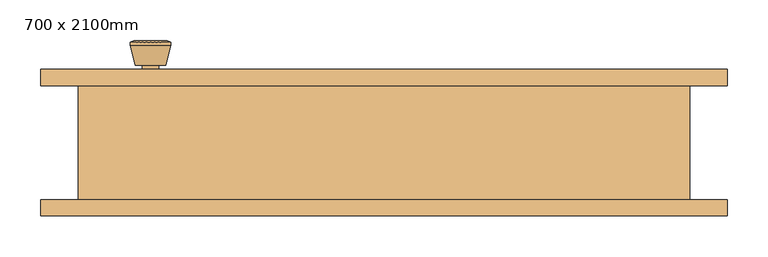
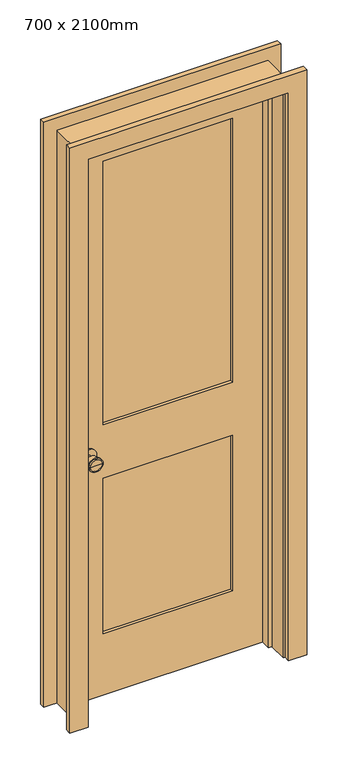
"""IFC4 building model written with IfcOpenShell, lengths in millimetres: door geometry, Porta-Interna-Única-2_Painel-Madeira : 700 x 2100mm."""

import ifcopenshell
import ifcopenshell.guid

model = None  # the IFC model being written
_history = None  # IfcOwnerHistory: only IFC2X3 demands one
_inside = {}  # id of a spatial element -> (the spatial element, [elements in it])
_under = {}  # id of a project, library or spatial element -> (it, [spatial elements below it])
_declared = {}  # id of a project -> (the project, [libraries it declares])
_typed = {}  # id of a type object -> (the type object, [elements of that type])
_made_of = {}  # id of a material, layer set ... -> (it, [elements and type objects made of it])


def new_model(schema):
    """Start an empty IFC model of exactly this schema.

    Asked for "IFC4X3", IfcOpenShell would pick the latest addendum, in which some entities
    have other attributes; the version numbers below select the first issue.
    IFC2X3 requires an IfcOwnerHistory on every rooted entity: one is made here for all.
    """
    global model, _history
    if schema == "IFC4X3":
        model = ifcopenshell.file(schema_version=(4, 3, 0, 0))
    else:
        model = ifcopenshell.file(schema=schema)
    _inside.clear()
    _under.clear()
    _declared.clear()
    _typed.clear()
    _made_of.clear()
    _history = None
    if model.schema == "IFC2X3":
        org = make("IfcOrganization", Name="unknown")
        user = make(
            "IfcPersonAndOrganization",
            ThePerson=make("IfcPerson", FamilyName="unknown"),
            TheOrganization=org,
        )
        app = make(
            "IfcApplication",
            ApplicationDeveloper=org,
            Version="unknown",
            ApplicationFullName="unknown",
            ApplicationIdentifier="unknown",
        )
        _history = make(
            "IfcOwnerHistory",
            OwningUser=user,
            OwningApplication=app,
            ChangeAction="ADDED",
            CreationDate=0,
        )
    return model


def make(cls, **values):
    """One entity of the class cls with the attributes given. An attribute that is None is left unset."""
    return model.create_entity(
        cls, **{name: value for name, value in values.items() if value is not None}
    )


def rooted(cls, **values):
    """An entity with a GlobalId (a new one), such as an element, a storey or a relation."""
    return make(cls, GlobalId=ifcopenshell.guid.new(), OwnerHistory=_history, **values)


def si_unit(unit_type, name, prefix=None):
    """IfcSIUnit, for example si_unit("LENGTHUNIT", "METRE", prefix="MILLI")."""
    return make("IfcSIUnit", UnitType=unit_type, Prefix=prefix, Name=name)


def assignment(units):
    """IfcUnitAssignment: the units of a project."""
    return None if units is None else make("IfcUnitAssignment", Units=units)


def point(xyz):
    """IfcCartesianPoint."""
    return None if xyz is None else make("IfcCartesianPoint", Coordinates=xyz)


def direction(xyz):
    """IfcDirection."""
    return None if xyz is None else make("IfcDirection", DirectionRatios=xyz)


def frame(location, z_axis=None, x_axis=None):
    """IfcAxis2Placement3D, a coordinate frame: its origin and axes. An axis left out is left unset."""
    return make(
        "IfcAxis2Placement3D",
        Location=point(location),
        Axis=direction(z_axis),
        RefDirection=direction(x_axis),
    )


def frame_2d(location, x_axis=None):
    """IfcAxis2Placement2D, a coordinate frame in the plane: its origin and x axis."""
    return make(
        "IfcAxis2Placement2D", Location=point(location), RefDirection=direction(x_axis)
    )


def origin():
    """The frame at (0, 0, 0) with its axes left unset."""
    return frame((0.0, 0.0, 0.0))


def place(relative_to, where):
    """IfcLocalPlacement: puts the frame where relative to a parent placement (None: the world)."""
    return make(
        "IfcLocalPlacement", PlacementRelTo=relative_to, RelativePlacement=where
    )


def context(
    kind, dimensions, precision=None, world=None, true_north=None, identifier=None
):
    """IfcGeometricRepresentationContext, for example the 3D "Model" context."""
    return make(
        "IfcGeometricRepresentationContext",
        ContextIdentifier=identifier,
        ContextType=kind,
        CoordinateSpaceDimension=dimensions,
        Precision=precision,
        WorldCoordinateSystem=world,
        TrueNorth=true_north,
    )


def project(units=None, contexts=None):
    """IfcProject with its units and contexts."""
    return rooted(
        "IfcProject",
        Name="project",
        RepresentationContexts=contexts,
        UnitsInContext=assignment(units),
    )


def spatial(cls, under=None, at=None, **own):
    """A site, building, storey or space (cls), placed at a placement, below another one or the project."""
    s = rooted(cls, ObjectPlacement=at, **own)
    if under is not None:
        _under.setdefault(under.id(), (under, []))[1].append(s)
    return s


def polyline(points):
    """IfcPolyline through the points."""
    return make("IfcPolyline", Points=[point(p) for p in points])


def circle_curve(where, radius):
    """IfcCircle in the frame where."""
    return make("IfcCircle", Position=where, Radius=radius)


def trimmed(basis, trim1, trim2, sense, master):
    """IfcTrimmedCurve: the piece of a basis curve between two trims."""
    return make(
        "IfcTrimmedCurve",
        BasisCurve=basis,
        Trim1=trim1,
        Trim2=trim2,
        SenseAgreement=sense,
        MasterRepresentation=master,
    )


def segment(curve, same_sense, transition):
    """IfcCompositeCurveSegment."""
    return make(
        "IfcCompositeCurveSegment",
        Transition=transition,
        SameSense=same_sense,
        ParentCurve=curve,
    )


def composite_curve(segments, self_intersect=None):
    """IfcCompositeCurve: segments joined end to end."""
    return make("IfcCompositeCurve", Segments=segments, SelfIntersect=self_intersect)


def outline(outer, holes=None, kind="AREA"):
    """IfcArbitraryClosedProfileDef: a profile drawn as a closed curve; with holes, ...WithVoids."""
    if holes is None:
        return make("IfcArbitraryClosedProfileDef", ProfileType=kind, OuterCurve=outer)
    return make(
        "IfcArbitraryProfileDefWithVoids",
        ProfileType=kind,
        OuterCurve=outer,
        InnerCurves=holes,
    )


def extrude(swept, where, along, depth):
    """IfcExtrudedAreaSolid: the profile swept, set in the frame where, extruded along a direction by depth."""
    return make(
        "IfcExtrudedAreaSolid",
        SweptArea=swept,
        Position=where,
        ExtrudedDirection=direction(along),
        Depth=depth,
    )


def faces_of(points, faces, orient=None, outer=None):
    """IfcFace entities. A face is a list of loops; a loop is a list of indices into points, from 0.

    orient and outer hold one flag for each loop. By default every Orientation is true, the
    first loop of a face is its IfcFaceOuterBound and the others are IfcFaceBound.
    """
    made = []
    for i, loops in enumerate(faces):
        bounds = []
        for j, loop in enumerate(loops):
            is_outer = j == 0 if outer is None else outer[i][j]
            bounds.append(
                make(
                    "IfcFaceOuterBound" if is_outer else "IfcFaceBound",
                    Bound=make("IfcPolyLoop", Polygon=[points[k] for k in loop]),
                    Orientation=True if orient is None else orient[i][j],
                )
            )
        made.append(make("IfcFace", Bounds=bounds))
    return made


def faceted_brep(points, faces, orient=None, outer=None, voids=None):
    """IfcFacetedBrep: a solid bounded by flat faces; with voids (closed shells), ...WithVoids."""
    shared = [point(p) for p in points]
    hull = make("IfcClosedShell", CfsFaces=faces_of(shared, faces, orient, outer))
    if voids is None:
        return make("IfcFacetedBrep", Outer=hull)
    return make(
        "IfcFacetedBrepWithVoids",
        Outer=hull,
        Voids=[
            make(cls, CfsFaces=faces_of(shared, fs, o, b)) for cls, fs, o, b in voids
        ],
    )


def shape(context_of_items, identifier, shape_type, items):
    """IfcShapeRepresentation: the items that make up one representation, for example the "Body"."""
    return make(
        "IfcShapeRepresentation",
        ContextOfItems=context_of_items,
        RepresentationIdentifier=identifier,
        RepresentationType=shape_type,
        Items=items,
    )


def source(mapping_origin, context_of_items, identifier, shape_type, items):
    """IfcRepresentationMap: a shape defined once, which mapped items show again and again."""
    return make(
        "IfcRepresentationMap",
        MappingOrigin=mapping_origin,
        MappedRepresentation=shape(context_of_items, identifier, shape_type, items),
    )


def transform(
    local_origin,
    x_axis=None,
    y_axis=None,
    z_axis=None,
    scale=None,
    scale2=None,
    scale3=None,
    uniform=True,
):
    """IfcCartesianTransformationOperator3D, or its non-uniform kind. x_axis, y_axis, z_axis: its Axis1, 2, 3."""
    if uniform:
        return make(
            "IfcCartesianTransformationOperator3D",
            Axis1=direction(x_axis),
            Axis2=direction(y_axis),
            LocalOrigin=point(local_origin),
            Scale=scale,
            Axis3=direction(z_axis),
        )
    return make(
        "IfcCartesianTransformationOperator3DnonUniform",
        Axis1=direction(x_axis),
        Axis2=direction(y_axis),
        LocalOrigin=point(local_origin),
        Scale=scale,
        Axis3=direction(z_axis),
        Scale2=scale2,
        Scale3=scale3,
    )


def mapped(mapping_source, mapping_target):
    """IfcMappedItem: shows the shape of a source again, moved by a transform."""
    return make(
        "IfcMappedItem", MappingSource=mapping_source, MappingTarget=mapping_target
    )


def made_of(thing, what):
    """Note that an element or type object is made of a material, layer set ...; save() writes the relation."""
    if what is not None:
        _made_of.setdefault(what.id(), (what, []))[1].append(thing)
    return thing


def element(
    cls,
    number,
    at=None,
    inside=None,
    cuts=None,
    type_object=None,
    material=None,
    context=None,
    identifier="Body",
    shape_type=None,
    held_by="IfcProductDefinitionShape",
    body=None,
    shapes=None,
    **own,
):
    """One element of the class cls, such as IfcWall. Its Tag is "e" and its number.

    at: its placement. inside: the storey or other place that contains it. cuts: it is an
    opening in that element (IfcRelVoidsElement). A single representation is given by context,
    identifier, shape_type and body (its items); several are given by shapes. held_by: the class
    of the entity that holds the representations. save() writes the other relations.
    """
    e = rooted(cls, Tag="e%d" % number, ObjectPlacement=at, **own)
    if body is not None:
        shapes = [shape(context, identifier, shape_type, body)]
    if shapes is not None:
        e.Representation = make(held_by, Representations=shapes)
    if inside is not None:
        _inside.setdefault(inside.id(), (inside, []))[1].append(e)
    if cuts is not None:
        rooted(
            "IfcRelVoidsElement", RelatingBuildingElement=cuts, RelatedOpeningElement=e
        )
    if type_object is not None:
        _typed.setdefault(type_object.id(), (type_object, []))[1].append(e)
    return made_of(e, material)


def aggregate(whole, parts):
    """IfcRelAggregates: a whole, such as a stair, and the parts it consists of."""
    return rooted("IfcRelAggregates", RelatingObject=whole, RelatedObjects=parts)


def save(model, path):
    """Write the relations noted so far, then the file.

    IfcRelAggregates (storeys below a building ...), IfcRelContainedInSpatialStructure (elements
    in a storey), IfcRelDefinesByType, IfcRelAssociatesMaterial and IfcRelDeclares: one each for
    every whole, place, type object, material and project.
    """
    for whole, parts in _under.values():
        aggregate(whole, parts)
    for where, things in _inside.values():
        rooted(
            "IfcRelContainedInSpatialStructure",
            RelatedElements=things,
            RelatingStructure=where,
        )
    for kind, things in _typed.values():
        rooted("IfcRelDefinesByType", RelatedObjects=things, RelatingType=kind)
    for what, things in _made_of.values():
        rooted("IfcRelAssociatesMaterial", RelatedObjects=things, RelatingMaterial=what)
    for by, libraries in _declared.values():
        rooted("IfcRelDeclares", RelatingContext=by, RelatedDefinitions=libraries)
    model.write(path)


def plane_surface(at):
    """IfcPlane: the flat surface through the origin of the frame at, square to its z axis."""
    return make("IfcPlane", Position=at)


def cylinder_surface(at, radius):
    """IfcCylindricalSurface: all points at the distance radius from the z axis of the frame at."""
    return make("IfcCylindricalSurface", Position=at, Radius=radius)


def revolved_surface(curve, axis_point, axis_direction):
    """IfcSurfaceOfRevolution: the curve turned about the line through axis_point along axis_direction."""
    return make(
        "IfcSurfaceOfRevolution",
        SweptCurve=make("IfcArbitraryOpenProfileDef", ProfileType="CURVE", Curve=curve),
        AxisPosition=make("IfcAxis1Placement", Location=point(axis_point), Axis=direction(axis_direction)),
    )


def advanced_brep(points, edges, surfaces, faces):
    """IfcAdvancedBrep: a solid bounded by faces that lie on surfaces and meet in shared edges.

    An edge is (start, end): straight between two places in points (the first is 0);
    or (start, end, curve); or (start, end, curve, False) where it runs against its curve.
    A face is (place in surfaces, loops), or (place, loops, False) where it looks against
    its surface's normal. A loop lists edges by number (the first is 1), with a minus sign
    where the edge is run from its end to its start. The first loop is the outer one.
    """
    corners = [point(p) for p in points]
    vertices = [make("IfcVertexPoint", VertexGeometry=c) for c in corners]
    made = []
    for start, end, *more in edges:
        made.append(
            make(
                "IfcEdgeCurve",
                EdgeStart=vertices[start],
                EdgeEnd=vertices[end],
                EdgeGeometry=more[0] if more else make("IfcPolyline", Points=[corners[start], corners[end]]),
                SameSense=more[1] if len(more) > 1 else True,
            )
        )
    hull = []
    for where, loops, *sense in faces:
        bounds = []
        for j, loop in enumerate(loops):
            ring = [make("IfcOrientedEdge", EdgeElement=made[abs(k) - 1], Orientation=k > 0) for k in loop]
            bounds.append(
                make(
                    "IfcFaceOuterBound" if j == 0 else "IfcFaceBound",
                    Bound=make("IfcEdgeLoop", EdgeList=ring),
                    Orientation=True,
                )
            )
        hull.append(make("IfcAdvancedFace", Bounds=bounds, FaceSurface=surfaces[where], SameSense=sense[0] if sense else True))
    return make("IfcAdvancedBrep", Outer=make("IfcClosedShell", CfsFaces=hull))


def door_700_x_2100mm_663e0b52(model_context):
    return source(origin(), model_context, "Body", "SolidModel", [
        advanced_brep(
        [(-286.5, 25.825, 914.4), (-276.5, 25.825, 914.4), (-296.5, 25.825, 914.4), (-266.0241324, -23.175, 914.4), (-286.5, -23.175, 914.4), (-306.9758676, -23.175, 914.4), (-261.5, -21.3471319, 914.4), (-311.5, -21.3471319, 914.4), (-261.5, -17.8834537, 914.4), (-311.5, -17.8834537, 914.4), (-267.863764, 6.825, 914.4), (-305.136236, 6.825, 914.4), (-276.5, 6.825, 914.4), (-296.5, 6.825, 914.4)],
        [
            (0, 1),
            (1, 2, circle_curve(frame((-286.5, 25.825, 914.4), z_axis=(0.0, 1.0, 0.0), x_axis=(-1.0, 0.0, 0.0)), 10.0)),
            (2, 0),
            (2, 1, circle_curve(frame((-286.5, 25.825, 914.4), z_axis=(0.0, 1.0, 0.0), x_axis=(-1.0, 0.0, 0.0)), 10.0)),
            (3, 4),
            (4, 5),
            (5, 3, circle_curve(frame((-286.5, -23.175, 914.4), z_axis=(0.0, -1.0, 0.0), x_axis=(-1.0, 0.0, 0.0)), 20.4758676)),
            (3, 5, circle_curve(frame((-286.5, -23.175, 914.4), z_axis=(0.0, -1.0, 0.0), x_axis=(-1.0, 0.0, 0.0)), 20.4758676)),
            (6, 3),
            (5, 7),
            (7, 6, circle_curve(frame((-286.5, -21.3471319, 914.4), z_axis=(0.0, -1.0, 0.0), x_axis=(-1.0, 0.0, 0.0)), 25.0)),
            (6, 7, circle_curve(frame((-286.5, -21.3471319, 914.4), z_axis=(0.0, -1.0, 0.0), x_axis=(-1.0, 0.0, 0.0)), 25.0)),
            (8, 6),
            (7, 9),
            (9, 8, circle_curve(frame((-286.5, -17.8834537, 914.4), z_axis=(0.0, -1.0, 0.0), x_axis=(-1.0, 0.0, 0.0)), 25.0)),
            (8, 9, circle_curve(frame((-286.5, -17.8834537, 914.4), z_axis=(0.0, -1.0, 0.0), x_axis=(-1.0, 0.0, 0.0)), 25.0)),
            (10, 8),
            (9, 11),
            (11, 10, circle_curve(frame((-286.5, 6.825, 914.4), z_axis=(0.0, -1.0, 0.0), x_axis=(-1.0, 0.0, 0.0)), 18.636236)),
            (10, 11, circle_curve(frame((-286.5, 6.825, 914.4), z_axis=(0.0, -1.0, 0.0), x_axis=(-1.0, 0.0, 0.0)), 18.636236)),
            (12, 10),
            (11, 13),
            (13, 12, circle_curve(frame((-286.5, 6.825, 914.4), z_axis=(0.0, -1.0, 0.0), x_axis=(-1.0, 0.0, 0.0)), 10.0)),
            (12, 13, circle_curve(frame((-286.5, 6.825, 914.4), z_axis=(0.0, -1.0, 0.0), x_axis=(-1.0, 0.0, 0.0)), 10.0)),
            (1, 12),
            (13, 2),
        ],
        [
            plane_surface(frame((-286.5, 25.825, 914.4), z_axis=(0.0, 1.0, 0.0), x_axis=(-1.0, 0.0, 0.0))),
            plane_surface(frame((-286.5, -23.175, 914.4), z_axis=(0.0, -1.0, 0.0), x_axis=(-1.0, 0.0, 0.0))),
            revolved_surface(polyline([(-306.9758676, -23.175, 914.4), (-311.5, -21.3471319, 914.4)]), (-286.5, 25.825, 914.4), (0.0, 1.0, 0.0)),
            cylinder_surface(frame((-286.5, 25.825, 914.4), z_axis=(0.0, 1.0, 0.0), x_axis=(-1.0, 0.0, 0.0)), 25.0),
            revolved_surface(polyline([(-311.5, -17.8834537, 914.4), (-305.136236, 6.825, 914.4)]), (-286.5, 25.825, 914.4), (0.0, 1.0, 0.0)),
            plane_surface(frame((-286.5, 6.825, 914.4), z_axis=(0.0, 1.0, 0.0), x_axis=(-1.0, 0.0, 0.0))),
            cylinder_surface(frame((-286.5, 25.825, 914.4), z_axis=(0.0, 1.0, 0.0), x_axis=(-1.0, 0.0, 0.0)), 10.0),
        ],
        [
            (0, [[1, 2, 3]]),
            (0, [[-3, 4, -1]]),
            (1, [[5, 6, 7]]),
            (1, [[-6, -5, 8]]),
            (2, [[9, -7, 10, 11]]),
            (2, [[-10, -8, -9, 12]]),
            (3, [[13, -11, 14, 15]]),
            (3, [[-14, -12, -13, 16]]),
            (4, [[17, -15, 18, 19]]),
            (4, [[-18, -16, -17, 20]]),
            (5, [[21, -19, 22, 23]]),
            (5, [[-22, -20, -21, 24]]),
            (6, [[25, -23, 26, -2]]),
            (6, [[-26, -24, -25, -4]]),
        ],
    ),
        extrude(outline(composite_curve([segment(trimmed(circle_curve(frame_2d((914.4, -286.5)), 30.0), [point((914.4, -316.5))], [point((914.4, -256.5))], False, "CARTESIAN"), True, "CONTINUOUS"), segment(trimmed(circle_curve(frame_2d((914.4, -286.5)), 30.0), [point((914.4, -256.5))], [point((914.4, -316.5))], False, "CARTESIAN"), True, "CONTINUOUS")], self_intersect=False)), frame((0.0, 25.825, 0.0), z_axis=(0.0, 1.0, 0.0), x_axis=(0.0, 0.0, 1.0)), (0.0, 0.0, 1.0), 6.0),
        advanced_brep(
        [(-286.5, 72.825, 914.4), (-296.5, 72.825, 914.4), (-276.5, 72.825, 914.4), (-266.0241324, 121.825, 914.4), (-306.9758676, 121.825, 914.4), (-286.5, 121.825, 914.4), (-261.5, 119.9971319, 914.4), (-311.5, 119.9971319, 914.4), (-261.5, 116.5334537, 914.4), (-311.5, 116.5334537, 914.4), (-267.863764, 91.825, 914.4), (-305.136236, 91.825, 914.4), (-276.5, 91.825, 914.4), (-296.5, 91.825, 914.4)],
        [
            (0, 1),
            (1, 2, circle_curve(frame((-286.5, 72.825, 914.4), z_axis=(0.0, -1.0, 0.0), x_axis=(-1.0, 0.0, 0.0)), 10.0)),
            (2, 0),
            (2, 1, circle_curve(frame((-286.5, 72.825, 914.4), z_axis=(0.0, -1.0, 0.0), x_axis=(-1.0, 0.0, 0.0)), 10.0)),
            (3, 4, circle_curve(frame((-286.5, 121.825, 914.4), z_axis=(0.0, 1.0, 0.0), x_axis=(-1.0, 0.0, 0.0)), 20.4758676)),
            (4, 5),
            (5, 3),
            (4, 3, circle_curve(frame((-286.5, 121.825, 914.4), z_axis=(0.0, 1.0, 0.0), x_axis=(-1.0, 0.0, 0.0)), 20.4758676)),
            (6, 7, circle_curve(frame((-286.5, 119.9971319, 914.4), z_axis=(0.0, 1.0, 0.0), x_axis=(-1.0, 0.0, 0.0)), 25.0)),
            (7, 4),
            (3, 6),
            (7, 6, circle_curve(frame((-286.5, 119.9971319, 914.4), z_axis=(0.0, 1.0, 0.0), x_axis=(-1.0, 0.0, 0.0)), 25.0)),
            (8, 9, circle_curve(frame((-286.5, 116.5334537, 914.4), z_axis=(0.0, 1.0, 0.0), x_axis=(-1.0, 0.0, 0.0)), 25.0)),
            (9, 7),
            (6, 8),
            (9, 8, circle_curve(frame((-286.5, 116.5334537, 914.4), z_axis=(0.0, 1.0, 0.0), x_axis=(-1.0, 0.0, 0.0)), 25.0)),
            (10, 11, circle_curve(frame((-286.5, 91.825, 914.4), z_axis=(0.0, 1.0, 0.0), x_axis=(-1.0, 0.0, 0.0)), 18.636236)),
            (11, 9),
            (8, 10),
            (11, 10, circle_curve(frame((-286.5, 91.825, 914.4), z_axis=(0.0, 1.0, 0.0), x_axis=(-1.0, 0.0, 0.0)), 18.636236)),
            (12, 13, circle_curve(frame((-286.5, 91.825, 914.4), z_axis=(0.0, 1.0, 0.0), x_axis=(-1.0, 0.0, 0.0)), 10.0)),
            (13, 11),
            (10, 12),
            (13, 12, circle_curve(frame((-286.5, 91.825, 914.4), z_axis=(0.0, 1.0, 0.0), x_axis=(-1.0, 0.0, 0.0)), 10.0)),
            (1, 13),
            (12, 2),
        ],
        [
            plane_surface(frame((-286.5, 72.825, 914.4), z_axis=(0.0, -1.0, 0.0), x_axis=(-1.0, 0.0, 0.0))),
            plane_surface(frame((-286.5, 121.825, 914.4), z_axis=(0.0, 1.0, 0.0), x_axis=(-1.0, 0.0, 0.0))),
            revolved_surface(polyline([(-306.9758676, 121.825, 914.4), (-311.5, 119.9971319, 914.4)]), (-286.5, 72.825, 914.4), (0.0, -1.0, 0.0)),
            cylinder_surface(frame((-286.5, 72.825, 914.4), z_axis=(0.0, -1.0, 0.0), x_axis=(-1.0, 0.0, 0.0)), 25.0),
            revolved_surface(polyline([(-311.5, 116.5334537, 914.4), (-305.136236, 91.825, 914.4)]), (-286.5, 72.825, 914.4), (0.0, -1.0, 0.0)),
            plane_surface(frame((-286.5, 91.825, 914.4), z_axis=(0.0, -1.0, 0.0), x_axis=(-1.0, 0.0, 0.0))),
            cylinder_surface(frame((-286.5, 72.825, 914.4), z_axis=(0.0, -1.0, 0.0), x_axis=(-1.0, 0.0, 0.0)), 10.0),
        ],
        [
            (0, [[1, 2, 3]]),
            (0, [[-3, 4, -1]]),
            (1, [[5, 6, 7]]),
            (1, [[8, -7, -6]]),
            (2, [[9, 10, -5, 11]]),
            (2, [[12, -11, -8, -10]]),
            (3, [[13, 14, -9, 15]]),
            (3, [[16, -15, -12, -14]]),
            (4, [[17, 18, -13, 19]]),
            (4, [[20, -19, -16, -18]]),
            (5, [[21, 22, -17, 23]]),
            (5, [[24, -23, -20, -22]]),
            (6, [[-2, 25, -21, 26]]),
            (6, [[-4, -26, -24, -25]]),
        ],
    ),
        extrude(outline(composite_curve([segment(trimmed(circle_curve(frame_2d((914.4, -286.5)), 30.0), [point((914.4, -316.5))], [point((914.4, -256.5))], False, "CARTESIAN"), True, "CONTINUOUS"), segment(trimmed(circle_curve(frame_2d((914.4, -286.5)), 30.0), [point((914.4, -256.5))], [point((914.4, -316.5))], False, "CARTESIAN"), True, "CONTINUOUS")], self_intersect=False)), frame((0.0, 66.825, 0.0), z_axis=(0.0, 1.0, 0.0), x_axis=(0.0, 0.0, 1.0)), (0.0, 0.0, 1.0), 6.0),
        extrude(outline(polyline([(230.0, 43.4916667), (-230.0, 43.4916667), (-230.0, 55.1583333), (230.0, 55.1583333), (230.0, 43.4916667)])), frame((0.0, 0.0, 1014.4), z_axis=(0.0, 0.0, 1.0), x_axis=(1.0, 0.0, 0.0)), (0.0, 0.0, 1.0), 990.6),
        extrude(outline(polyline([(230.0, 43.4916667), (-230.0, 43.4916667), (-230.0, 55.1583333), (230.0, 55.1583333), (230.0, 43.4916667)])), frame((0.0, 0.0, 230.0), z_axis=(0.0, 0.0, 1.0), x_axis=(1.0, 0.0, 0.0)), (0.0, 0.0, 1.0), 584.4),
        extrude(outline(polyline([(2125.0, -350.0), (0.0, -350.0), (0.0, 350.0), (2125.0, 350.0), (2125.0, -350.0)]), holes=[polyline([(2005.0, -230.0), (2005.0, 230.0), (1014.4, 230.0), (1014.4, -230.0), (2005.0, -230.0)]), polyline([(814.4, -230.0), (814.4, 230.0), (230.0, 230.0), (230.0, -230.0), (814.4, -230.0)])]), frame((0.0, 31.825, 0.0), z_axis=(0.0, 1.0, 0.0), x_axis=(0.0, 0.0, 1.0)), (0.0, 0.0, 1.0), 35.0),
        faceted_brep([(375.0, 66.825, 0.0), (375.0, -73.175, 0.0), (350.0, -73.175, 0.0), (350.0, -3.1, 0.0), (337.3, -3.1, 0.0), (337.3, 31.825, 0.0), (350.0, 31.825, 0.0), (350.0, 66.825, 0.0), (375.0, 66.825, 2150.0), (375.0, -73.175, 2150.0), (-375.0, -73.175, 2150.0), (-375.0, -73.175, 0.0), (-350.0, -73.175, 0.0), (-350.0, -73.175, 2125.0), (350.0, -73.175, 2125.0), (350.0, -3.1, 2125.0), (-350.0, -3.1, 2125.0), (-350.0, -3.1, 0.0), (-337.3, -3.1, 0.0), (-337.3, -3.1, 2112.3), (337.3, -3.1, 2112.3), (337.3, 31.825, 2112.3), (-337.3, 31.825, 2112.3), (-337.3, 31.825, 0.0), (-350.0, 31.825, 0.0), (-350.0, 31.825, 2125.0), (350.0, 31.825, 2125.0), (350.0, 66.825, 2125.0), (-350.0, 66.825, 2125.0), (-350.0, 66.825, 0.0), (-375.0, 66.825, 0.0), (-375.0, 66.825, 2150.0)], [[[0, 1, 2, 3, 4, 5, 6, 7]], [[1, 0, 8, 9]], [[2, 1, 9, 10, 11, 12, 13, 14]], [[3, 2, 14, 15]], [[4, 3, 15, 16, 17, 18, 19, 20]], [[5, 4, 20, 21]], [[6, 5, 21, 22, 23, 24, 25, 26]], [[7, 6, 26, 27]], [[0, 7, 27, 28, 29, 30, 31, 8]], [[9, 8, 31, 10]], [[15, 14, 13, 16]], [[21, 20, 19, 22]], [[27, 26, 25, 28]], [[30, 29, 24, 23, 18, 17, 12, 11]], [[10, 31, 30, 11]], [[16, 13, 12, 17]], [[22, 19, 18, 23]], [[28, 25, 24, 29]]]),
        extrude(outline(polyline([(0.0, 356.35), (0.0, 421.35), (2196.35, 421.35), (2196.35, -421.35), (0.0, -421.35), (0.0, -356.35), (2131.35, -356.35), (2131.35, 356.35), (0.0, 356.35)])), frame((0.0, -93.175, 0.0), z_axis=(0.0, 1.0, 0.0), x_axis=(0.0, 0.0, 1.0)), (0.0, 0.0, 1.0), 20.0),
        extrude(outline(polyline([(0.0, 356.35), (0.0, 421.35), (2196.35, 421.35), (2196.35, -421.35), (0.0, -421.35), (0.0, -356.35), (2131.35, -356.35), (2131.35, 356.35), (0.0, 356.35)])), frame((0.0, 66.825, 0.0), z_axis=(0.0, 1.0, 0.0), x_axis=(0.0, 0.0, 1.0)), (0.0, 0.0, 1.0), 20.0),
    ])


if __name__ == "__main__":
    model = new_model("IFC4")
    model_context = context("Model", 3, world=origin())
    ifc_project = project(units=[si_unit("LENGTHUNIT", "METRE", prefix="MILLI")], contexts=[model_context])
    site = spatial("IfcSite", under=ifc_project)
    building = spatial("IfcBuilding", under=site)
    placement = place(None, origin())
    door_700_x_2100mm_shape = door_700_x_2100mm_663e0b52(model_context)
    element("IfcDoor", 1, ObjectType="Porta-Interna-Única-2_Painel-Madeira : 700 x 2100mm", at=placement, inside=building, context=model_context, shape_type="MappedRepresentation", body=[
        mapped(door_700_x_2100mm_shape, transform((0.0, 0.0, 0.0), x_axis=(1.0, 0.0, 0.0), y_axis=(0.0, 1.0, 0.0), z_axis=(0.0, 0.0, 1.0))),
    ])
    save(model, "model.ifc")

# Revit data of these elements
# Type "Porta-Interna-Única-2_Painel-Madeira : 700 x 2100mm"
#   Type Mark = "141"
#   Assembly Code = "C1020300"
#   Analytic Construction = "Madeira"
#   Corrimão superior = 0.120 m
#   Thickness = 0.035 m
#   Thermal Resistance (R) = 0.455703 (m²·K)/W
#   Ângulo de abertura [instance default] = 90.00°
#   Estilos = 0.120 m
#   Rough Width = 0.750 m
#   Rough Height = 2.150 m
#   Bloquear corrimão = 0.200 m
#   Height = 2.125 m
#   Width = 0.700 m
#   Heat Transfer Coefficient (U) = 2.19465 W/(m²·K)
#   Corrimão inferior = 0.230 m
#   Material da apara = Cerejeira
#   Material do painel = Cerejeira
#   Material da moldura = Cerejeira
#   Material da maçaneta = Alumín. 1
#   Visual Light Transmittance = 0
#   Solar Heat Gain Coefficient = 0
#   Wall Closure = (empty or 0)
#   Function = (empty or 0)
# Element 1 (IfcDoor, "Porta-Interna-Única-2_Painel-Madeira : 700 x 2100mm")
#   Materials on its faces: "Cerejeira", "Alumín. 1"
# Materials
#   "Cerejeira": class "Madeira", colour RGB 226 177 128, transparency 0, Description = "Prunus Serotina", Cost = 0
#   "Alumín. 1": class "Metal", colour RGB 247 247 247, transparency 0, Description = "Alumín. 6061", Cost = 0
